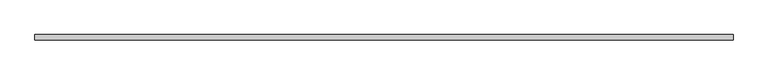
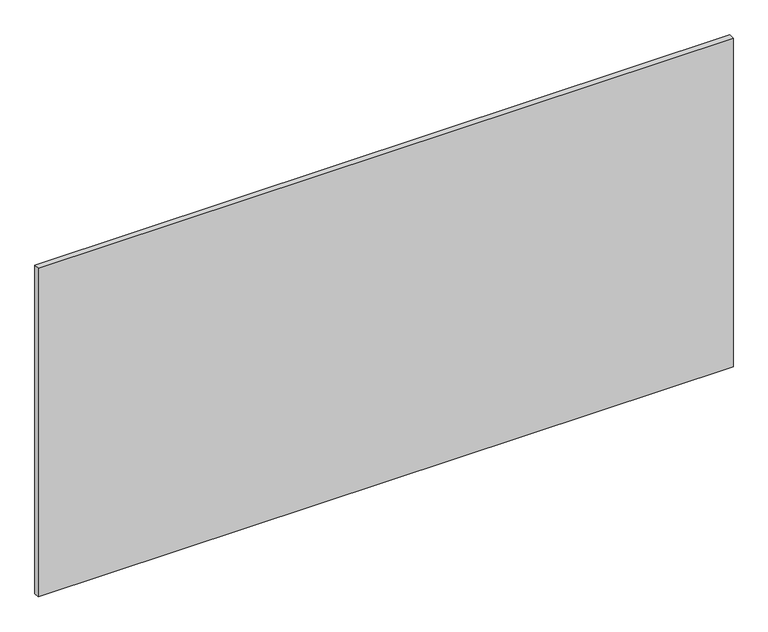
"""IFC4 building model written with IfcOpenShell, lengths in millimetres: proxy geometry, Inner panel:Inner panel:1:Inner panel:1 : Inner panel:Inner panel:300324:300043:Inner panel:1:Inner panel:1 : Inner panel:Inner panel:300324:300043 : Inner panel:Inner panel:1:Inner panel:1 : Inner panel:Inner panel:300324:300043:24 : Inner panel:Inner panel:1:Inner panel:1 : Inner panel:Inner panel:300324:300043:Inner panel:1:Inner panel:1 : Inner panel:Inner panel:300324:300043 : Inner panel:Inner panel:1:Inner panel:1 : Inner panel:Inner panel:300324:300043:300031."""

from ifc_helpers import new_model, si_unit, frame, origin, place, context, project, spatial, polyline, outline, extrude, source, transform, mapped, element, save


def generic_models_1fe94dea(model_context):
    return source(origin(), model_context, "Body", "SweptSolid", [
        extrude(outline(polyline([(594957.2867242, -567913.5913841), (597395.6867242, -567913.5913841), (597395.6867242, -567932.6413841), (594957.2867242, -567932.6413841), (594957.2867242, -567913.5913841)])), frame((0.0, 0.0, 3721.1), z_axis=(0.0, 0.0, 1.0), x_axis=(1.0, 0.0, 0.0)), (0.0, 0.0, 1.0), 1219.2),
    ])


if __name__ == "__main__":
    model = new_model("IFC4")
    model_context = context("Model", 3, world=origin())
    ifc_project = project(units=[si_unit("LENGTHUNIT", "METRE", prefix="MILLI")], contexts=[model_context])
    site = spatial("IfcSite", under=ifc_project)
    building = spatial("IfcBuilding", under=site)
    placement = place(None, origin())
    generic_models_shape = generic_models_1fe94dea(model_context)
    element("IfcBuildingElementProxy", 1, Name="Inner panel:Inner panel:1:Inner panel:1 : Inner panel:Inner panel:300324:300043:Inner panel:1:Inner panel:1 : Inner panel:Inner panel:300324:300043 : Inner panel:Inner panel:1:Inner panel:1 : Inner panel:Inner panel:300324:300043:24 : Inner panel:Inner panel:1:Inner panel:1 : Inner panel:Inner panel:300324:300043:Inner panel:1:Inner panel:1 : Inner panel:Inner panel:300324:300043 : Inner panel:Inner panel:1:Inner panel:1 : Inner panel:Inner panel:300324:300043:300031", ObjectType="Inner panel:Inner panel:1:Inner panel:1 : Inner panel:Inner panel:300324:300043:Inner panel:1:Inner panel:1 : Inner panel:Inner panel:300324:300043 : Inner panel:Inner panel:1:Inner panel:1 : Inner panel:Inner panel:300324:300043:24 : Inner panel:Inner panel:1:Inner panel:1 : Inner panel:Inner panel:300324:300043:Inner panel:1:Inner panel:1 : Inner panel:Inner panel:300324:300043 : Inner panel:Inner panel:1:Inner panel:1 : Inner panel:Inner panel:300324:300043:300031", at=placement, inside=building, context=model_context, shape_type="MappedRepresentation", body=[
        mapped(generic_models_shape, transform((0.0, 0.0, 0.0), x_axis=(1.0, 0.0, 0.0), y_axis=(0.0, 1.0, 0.0), z_axis=(0.0, 0.0, 1.0))),
    ])
    save(model, "model.ifc")

# Revit data of these elements
# Type "Inner panel:Inner panel:1:Inner panel:1 : Inner panel:Inner panel:300324:300043:Inner panel:1:Inner panel:1 : Inner panel:Inner panel:300324:300043 : Inner panel:Inner panel:1:Inner panel:1 : Inner panel:Inner panel:300324:300043:24 : Inner panel:Inner panel:1:Inner panel:1 : Inner panel:Inner panel:300324:300043:Inner panel:1:Inner panel:1 : Inner panel:Inner panel:300324:300043 : Inner panel:Inner panel:1:Inner panel:1 : Inner panel:Inner panel:300324:300043:300031"
#   NameOverride = "Inner panel:Inner panel:1:Inner panel:1 : Inner panel:Inner panel:300324:300043:Inner panel:1:Inner panel:1 : Inner panel:Inner panel:300324:300043 : Inner panel:Inner panel:1:Inner panel:1 : Inner panel:Inner panel:300324:300043:300031"
#   ObjectTypeOverride = "Inner panel:1:Inner panel:1 : Inner panel:Inner panel:300324:300043 : Inner panel:Inner panel:1:Inner panel:1 : Inner panel:Inner panel:300324:300043"
#   Reference = "Inner panel"
#   Tag = "300031"
# Element 1 (IfcBuildingElementProxy, "Inner panel:Inner panel:1:Inner panel:1 : Inner panel:Inner panel:300324:300043:Inner panel:1:Inner panel:1 : Inner panel:Inner panel:300324:300043 : Inner panel:Inner panel:1:Inner panel:1 : Inner panel:Inner panel:300324:300043:24 : Inner panel:Inner panel:1:Inner panel:1 : Inner panel:Inner panel:300324:300043:Inner panel:1:Inner panel:1 : Inner panel:Inner panel:300324:300043 : Inner panel:Inner panel:1:Inner panel:1 : Inner panel:Inner panel:300324:300043:300031")
#   Materials on its faces: "¾” (CLASS A) FIRE RETARDANT PLYWOOD ...OR… IF 1/4\" GYP. BD UNDER PLYWOOD, FLAME SPREAD TO BE CLASS C -  (FINISH: GRADE B - PREFINISHED STAINED/SEALED) - 1/4\" GAP BTWN PANELS (FASTENERS T.B.D.)"
# Materials
#   "¾” (CLASS A) FIRE RETARDANT PLYWOOD ...OR… IF 1/4\" GYP. BD UNDER PLYWOOD, FLAME SPREAD TO BE CLASS C -  (FINISH: GRADE B - PREFINISHED STAINED/SEALED) - 1/4\" GAP BTWN PANELS (FASTENERS T.B.D.)": class "Wood", colour RGB 149 120 74, transparency 0, Description = "Plywood, sheathing grade", Cost = 0
